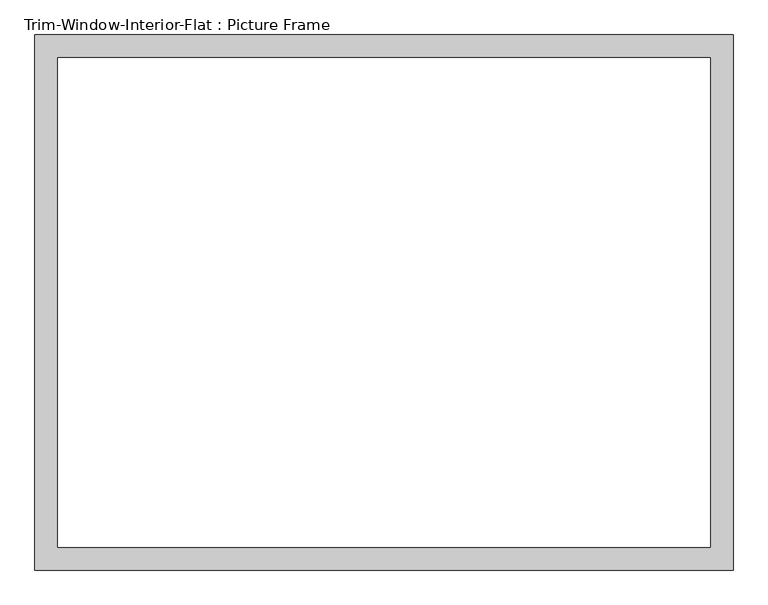
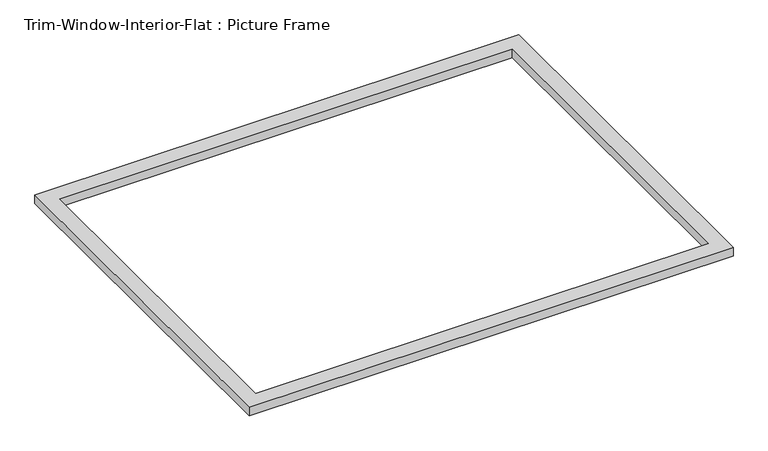
"""IFC4 building model written with IfcOpenShell, lengths in millimetres: proxy geometry, Trim-Window-Interior-Flat : Picture Frame."""

import ifcopenshell
import ifcopenshell.guid

model = None  # the IFC model being written
_history = None  # IfcOwnerHistory: only IFC2X3 demands one
_inside = {}  # id of a spatial element -> (the spatial element, [elements in it])
_under = {}  # id of a project, library or spatial element -> (it, [spatial elements below it])
_declared = {}  # id of a project -> (the project, [libraries it declares])
_typed = {}  # id of a type object -> (the type object, [elements of that type])
_made_of = {}  # id of a material, layer set ... -> (it, [elements and type objects made of it])


def new_model(schema):
    """Start an empty IFC model of exactly this schema.

    Asked for "IFC4X3", IfcOpenShell would pick the latest addendum, in which some entities
    have other attributes; the version numbers below select the first issue.
    IFC2X3 requires an IfcOwnerHistory on every rooted entity: one is made here for all.
    """
    global model, _history
    if schema == "IFC4X3":
        model = ifcopenshell.file(schema_version=(4, 3, 0, 0))
    else:
        model = ifcopenshell.file(schema=schema)
    _inside.clear()
    _under.clear()
    _declared.clear()
    _typed.clear()
    _made_of.clear()
    _history = None
    if model.schema == "IFC2X3":
        org = make("IfcOrganization", Name="unknown")
        user = make(
            "IfcPersonAndOrganization",
            ThePerson=make("IfcPerson", FamilyName="unknown"),
            TheOrganization=org,
        )
        app = make(
            "IfcApplication",
            ApplicationDeveloper=org,
            Version="unknown",
            ApplicationFullName="unknown",
            ApplicationIdentifier="unknown",
        )
        _history = make(
            "IfcOwnerHistory",
            OwningUser=user,
            OwningApplication=app,
            ChangeAction="ADDED",
            CreationDate=0,
        )
    return model


def make(cls, **values):
    """One entity of the class cls with the attributes given. An attribute that is None is left unset."""
    return model.create_entity(
        cls, **{name: value for name, value in values.items() if value is not None}
    )


def rooted(cls, **values):
    """An entity with a GlobalId (a new one), such as an element, a storey or a relation."""
    return make(cls, GlobalId=ifcopenshell.guid.new(), OwnerHistory=_history, **values)


def si_unit(unit_type, name, prefix=None):
    """IfcSIUnit, for example si_unit("LENGTHUNIT", "METRE", prefix="MILLI")."""
    return make("IfcSIUnit", UnitType=unit_type, Prefix=prefix, Name=name)


def assignment(units):
    """IfcUnitAssignment: the units of a project."""
    return None if units is None else make("IfcUnitAssignment", Units=units)


def point(xyz):
    """IfcCartesianPoint."""
    return None if xyz is None else make("IfcCartesianPoint", Coordinates=xyz)


def direction(xyz):
    """IfcDirection."""
    return None if xyz is None else make("IfcDirection", DirectionRatios=xyz)


def frame(location, z_axis=None, x_axis=None):
    """IfcAxis2Placement3D, a coordinate frame: its origin and axes. An axis left out is left unset."""
    return make(
        "IfcAxis2Placement3D",
        Location=point(location),
        Axis=direction(z_axis),
        RefDirection=direction(x_axis),
    )


def origin():
    """The frame at (0, 0, 0) with its axes left unset."""
    return frame((0.0, 0.0, 0.0))


def origin_with_axes():
    """The frame at (0, 0, 0) with the z axis (0, 0, 1) and the x axis (1, 0, 0) written out."""
    return frame((0.0, 0.0, 0.0), z_axis=(0.0, 0.0, 1.0), x_axis=(1.0, 0.0, 0.0))


def place(relative_to, where):
    """IfcLocalPlacement: puts the frame where relative to a parent placement (None: the world)."""
    return make(
        "IfcLocalPlacement", PlacementRelTo=relative_to, RelativePlacement=where
    )


def context(
    kind, dimensions, precision=None, world=None, true_north=None, identifier=None
):
    """IfcGeometricRepresentationContext, for example the 3D "Model" context."""
    return make(
        "IfcGeometricRepresentationContext",
        ContextIdentifier=identifier,
        ContextType=kind,
        CoordinateSpaceDimension=dimensions,
        Precision=precision,
        WorldCoordinateSystem=world,
        TrueNorth=true_north,
    )


def project(units=None, contexts=None):
    """IfcProject with its units and contexts."""
    return rooted(
        "IfcProject",
        Name="project",
        RepresentationContexts=contexts,
        UnitsInContext=assignment(units),
    )


def spatial(cls, under=None, at=None, **own):
    """A site, building, storey or space (cls), placed at a placement, below another one or the project."""
    s = rooted(cls, ObjectPlacement=at, **own)
    if under is not None:
        _under.setdefault(under.id(), (under, []))[1].append(s)
    return s


def polyline(points):
    """IfcPolyline through the points."""
    return make("IfcPolyline", Points=[point(p) for p in points])


def outline(outer, holes=None, kind="AREA"):
    """IfcArbitraryClosedProfileDef: a profile drawn as a closed curve; with holes, ...WithVoids."""
    if holes is None:
        return make("IfcArbitraryClosedProfileDef", ProfileType=kind, OuterCurve=outer)
    return make(
        "IfcArbitraryProfileDefWithVoids",
        ProfileType=kind,
        OuterCurve=outer,
        InnerCurves=holes,
    )


def extrude(swept, where, along, depth):
    """IfcExtrudedAreaSolid: the profile swept, set in the frame where, extruded along a direction by depth."""
    return make(
        "IfcExtrudedAreaSolid",
        SweptArea=swept,
        Position=where,
        ExtrudedDirection=direction(along),
        Depth=depth,
    )


def shape(context_of_items, identifier, shape_type, items):
    """IfcShapeRepresentation: the items that make up one representation, for example the "Body"."""
    return make(
        "IfcShapeRepresentation",
        ContextOfItems=context_of_items,
        RepresentationIdentifier=identifier,
        RepresentationType=shape_type,
        Items=items,
    )


def source(mapping_origin, context_of_items, identifier, shape_type, items):
    """IfcRepresentationMap: a shape defined once, which mapped items show again and again."""
    return make(
        "IfcRepresentationMap",
        MappingOrigin=mapping_origin,
        MappedRepresentation=shape(context_of_items, identifier, shape_type, items),
    )


def transform(
    local_origin,
    x_axis=None,
    y_axis=None,
    z_axis=None,
    scale=None,
    scale2=None,
    scale3=None,
    uniform=True,
):
    """IfcCartesianTransformationOperator3D, or its non-uniform kind. x_axis, y_axis, z_axis: its Axis1, 2, 3."""
    if uniform:
        return make(
            "IfcCartesianTransformationOperator3D",
            Axis1=direction(x_axis),
            Axis2=direction(y_axis),
            LocalOrigin=point(local_origin),
            Scale=scale,
            Axis3=direction(z_axis),
        )
    return make(
        "IfcCartesianTransformationOperator3DnonUniform",
        Axis1=direction(x_axis),
        Axis2=direction(y_axis),
        LocalOrigin=point(local_origin),
        Scale=scale,
        Axis3=direction(z_axis),
        Scale2=scale2,
        Scale3=scale3,
    )


def mapped(mapping_source, mapping_target):
    """IfcMappedItem: shows the shape of a source again, moved by a transform."""
    return make(
        "IfcMappedItem", MappingSource=mapping_source, MappingTarget=mapping_target
    )


def made_of(thing, what):
    """Note that an element or type object is made of a material, layer set ...; save() writes the relation."""
    if what is not None:
        _made_of.setdefault(what.id(), (what, []))[1].append(thing)
    return thing


def element(
    cls,
    number,
    at=None,
    inside=None,
    cuts=None,
    type_object=None,
    material=None,
    context=None,
    identifier="Body",
    shape_type=None,
    held_by="IfcProductDefinitionShape",
    body=None,
    shapes=None,
    **own,
):
    """One element of the class cls, such as IfcWall. Its Tag is "e" and its number.

    at: its placement. inside: the storey or other place that contains it. cuts: it is an
    opening in that element (IfcRelVoidsElement). A single representation is given by context,
    identifier, shape_type and body (its items); several are given by shapes. held_by: the class
    of the entity that holds the representations. save() writes the other relations.
    """
    e = rooted(cls, Tag="e%d" % number, ObjectPlacement=at, **own)
    if body is not None:
        shapes = [shape(context, identifier, shape_type, body)]
    if shapes is not None:
        e.Representation = make(held_by, Representations=shapes)
    if inside is not None:
        _inside.setdefault(inside.id(), (inside, []))[1].append(e)
    if cuts is not None:
        rooted(
            "IfcRelVoidsElement", RelatingBuildingElement=cuts, RelatedOpeningElement=e
        )
    if type_object is not None:
        _typed.setdefault(type_object.id(), (type_object, []))[1].append(e)
    return made_of(e, material)


def aggregate(whole, parts):
    """IfcRelAggregates: a whole, such as a stair, and the parts it consists of."""
    return rooted("IfcRelAggregates", RelatingObject=whole, RelatedObjects=parts)


def save(model, path):
    """Write the relations noted so far, then the file.

    IfcRelAggregates (storeys below a building ...), IfcRelContainedInSpatialStructure (elements
    in a storey), IfcRelDefinesByType, IfcRelAssociatesMaterial and IfcRelDeclares: one each for
    every whole, place, type object, material and project.
    """
    for whole, parts in _under.values():
        aggregate(whole, parts)
    for where, things in _inside.values():
        rooted(
            "IfcRelContainedInSpatialStructure",
            RelatedElements=things,
            RelatingStructure=where,
        )
    for kind, things in _typed.values():
        rooted("IfcRelDefinesByType", RelatedObjects=things, RelatingType=kind)
    for what, things in _made_of.values():
        rooted("IfcRelAssociatesMaterial", RelatedObjects=things, RelatingMaterial=what)
    for by, libraries in _declared.values():
        rooted("IfcRelDeclares", RelatingContext=by, RelatedDefinitions=libraries)
    model.write(path)


def trim_window_interior_flat_picture_frame_4bb1ca52(model_context):
    return source(origin(), model_context, "Body", "SweptSolid", [
        extrude(outline(polyline([(869.95, 44.45), (869.95, -1289.05), (-869.95, -1289.05), (-869.95, 44.45), (869.95, 44.45)]), holes=[polyline([(812.8, -12.7), (-812.8, -12.7), (-812.8, -1231.9), (812.8, -1231.9), (812.8, -12.7)])]), origin_with_axes(), (0.0, 0.0, 1.0), 31.75),
    ])


if __name__ == "__main__":
    model = new_model("IFC4")
    model_context = context("Model", 3, world=origin())
    ifc_project = project(units=[si_unit("LENGTHUNIT", "METRE", prefix="MILLI")], contexts=[model_context])
    site = spatial("IfcSite", under=ifc_project)
    building = spatial("IfcBuilding", under=site)
    placement = place(None, origin())
    trim_window_interior_flat_picture_frame_shape = trim_window_interior_flat_picture_frame_4bb1ca52(model_context)
    element("IfcBuildingElementProxy", 1, Name="Trim-Window-Interior-Flat : Picture Frame", ObjectType="Trim-Window-Interior-Flat : Picture Frame", at=placement, inside=building, context=model_context, shape_type="MappedRepresentation", body=[
        mapped(trim_window_interior_flat_picture_frame_shape, transform((0.0, 0.0, 0.0), x_axis=(1.0, 0.0, 0.0), y_axis=(0.0, 1.0, 0.0), z_axis=(0.0, 0.0, 1.0))),
    ])
    save(model, "model.ifc")

# Revit data of these elements
# Type "Trim-Window-Interior-Flat : Picture Frame"
#   Trim Thickness_Picture Frame = 0' - 1 1/4"
#   Trim Width = 0' - 2 1/4"
#   Trim Thickness_with Sill = 0' - 0 3/4"
#   Sill Thickness = 0' - 1 1/4"
#   Opening Width [instance default] = 2' - 0"
#   Opening Height [instance default] = 3' - 0"
#   Default Elevation = 4' - 0"
#   Sill = no
#   Picture Frame = yes
#   Trim Material [instance default] = none
# Element 1 (IfcBuildingElementProxy, "Trim-Window-Interior-Flat : Picture Frame")
#   Opening Width = 5' - 5"
#   Opening Height = 4' - 1"
#   Trim Material = Wood - Stained
#   Materials on its faces: "Wood - Stained"
# Materials
#   "Wood - Stained": class "Wood", colour RGB 224 178 126, transparency 0, Cost = 0
